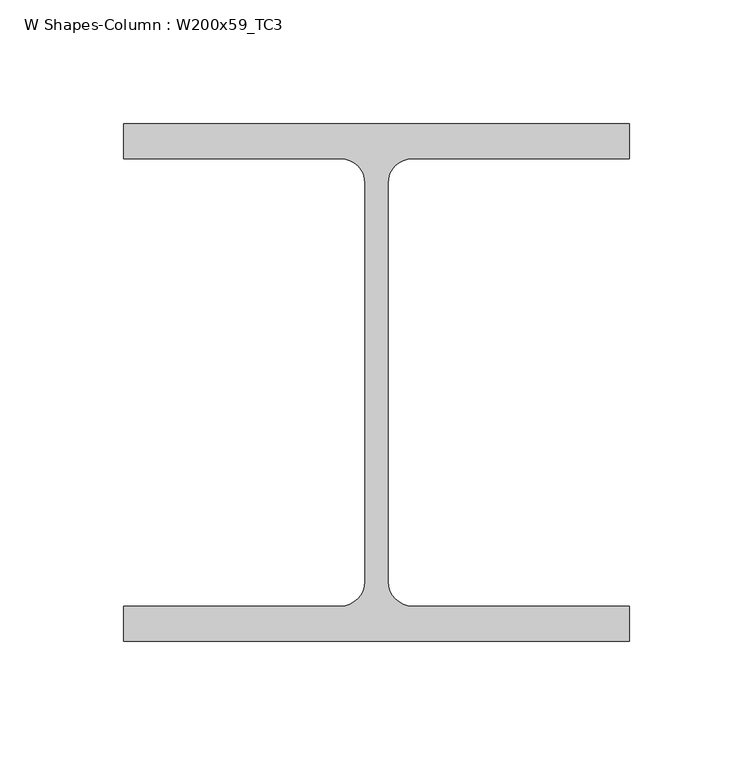
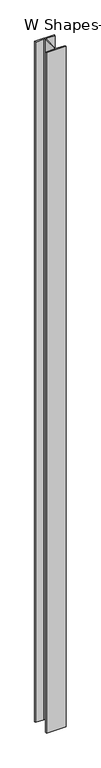
"""IFC4 building model written with IfcOpenShell, lengths in millimetres: column geometry, W Shapes-Column : W200x59_TC3."""

from ifc_helpers import new_model, si_unit, point, frame, frame_2d, origin, place, context, project, spatial, polyline, circle_curve, trimmed, segment, composite_curve, outline, extrude, source, transform, mapped, element, save


def w_shapes_column_w200x59_tc3_7e99c75d(model_context):
    return source(origin(), model_context, "Body", "SweptSolid", [
        extrude(outline(composite_curve([segment(polyline([(102.489, 104.775), (102.489, 90.551), (14.5796, 90.551)]), True, "CONTINUOUS"), segment(trimmed(circle_curve(frame_2d((14.5796, 80.5434)), 10.0076), [point((14.5796, 90.551))], [point((4.572, 80.5434))], True, "CARTESIAN"), True, "CONTINUOUS"), segment(polyline([(4.572, 80.5434), (4.572, -80.5434)]), True, "CONTINUOUS"), segment(trimmed(circle_curve(frame_2d((14.5796, -80.5434)), 10.0076), [point((4.572, -80.5434))], [point((14.5796, -90.551))], True, "CARTESIAN"), True, "CONTINUOUS"), segment(polyline([(14.5796, -90.551), (102.489, -90.551), (102.489, -104.775), (-102.489, -104.775), (-102.489, -90.551), (-14.5796, -90.551)]), True, "CONTINUOUS"), segment(trimmed(circle_curve(frame_2d((-14.5796, -80.5434)), 10.0076), [point((-14.5796, -90.551))], [point((-4.572, -80.5434))], True, "CARTESIAN"), True, "CONTINUOUS"), segment(polyline([(-4.572, -80.5434), (-4.572, 80.5434)]), True, "CONTINUOUS"), segment(trimmed(circle_curve(frame_2d((-14.5796, 80.5434)), 10.0076), [point((-4.572, 80.5434))], [point((-14.5796, 90.551))], True, "CARTESIAN"), True, "CONTINUOUS"), segment(polyline([(-14.5796, 90.551), (-102.489, 90.551), (-102.489, 104.775), (102.489, 104.775)]), True, "CONTINUOUS")], self_intersect=False)), frame((0.0, 0.0, 200.0), z_axis=(0.0, 0.0, 1.0), x_axis=(1.0, 0.0, 0.0)), (0.0, 0.0, 1.0), 7500.0),
    ])


if __name__ == "__main__":
    model = new_model("IFC4")
    model_context = context("Model", 3, world=origin())
    ifc_project = project(units=[si_unit("LENGTHUNIT", "METRE", prefix="MILLI")], contexts=[model_context])
    site = spatial("IfcSite", under=ifc_project)
    building = spatial("IfcBuilding", under=site)
    placement = place(None, origin())
    w_shapes_column_w200x59_tc3_shape = w_shapes_column_w200x59_tc3_7e99c75d(model_context)
    element("IfcColumn", 1, ObjectType="W Shapes-Column : W200x59_TC3", at=placement, inside=building, context=model_context, shape_type="MappedRepresentation", body=[
        mapped(w_shapes_column_w200x59_tc3_shape, transform((0.0, 0.0, 0.0), x_axis=(1.0, 0.0, 0.0), y_axis=(0.0, 1.0, 0.0), z_axis=(0.0, 0.0, 1.0))),
    ])
    save(model, "model.ifc")

# Revit data of these elements
# Type "W Shapes-Column : W200x59_TC3"
#   Section Name Key = "W8X40"
#   Assembly Code = "B10"
#   Width = 20.4978 cm
#   Web Thickness = 0.9144 cm
#   Web Fillet = 1.0008 cm
#   Warping Constant = 194957.0 cm⁶
#   Torsional Moment of Inertia = 46.6179 cm⁴
#   Section Area = 75.4837 cm²
#   Plastic Modulus weak axis = 303.161 cm³
#   Plastic Modulus strong axis = 652.205 cm³
#   Perimeter = 1.20396 m²/m
#   Nominal Weight = 59.5266 kgf/m
#   Moment of Inertia weak axis = 2043.70 cm⁴
#   Moment of Inertia strong axis = 6076.98 cm⁴
#   Height = 20.955 cm
#   Flange Thickness = 1.4224 cm
#   Elastic Modulus weak axis = 199.922 cm³
#   Elastic Modulus strong axis = 581.741 cm³
#   Clear Web Height = 14.605 cm
#   Centroid Vertical = 10.4775 cm
#   Centroid Horizontal = 10.2489 cm
#   Bolt Spacing = 13.97 cm
#   Structural Material [instance default] = Steel ASTM A992
#   Principal Axes Angle = 0
# Element 1 (IfcColumn, "W Shapes-Column : W200x59_TC3")
#   Structural Material = none
# Materials
#   "Steel ASTM A992": class "Metal", colour RGB 199 199 199, transparency 0, Description = "Structural steel 50ksi", Cost = 0
